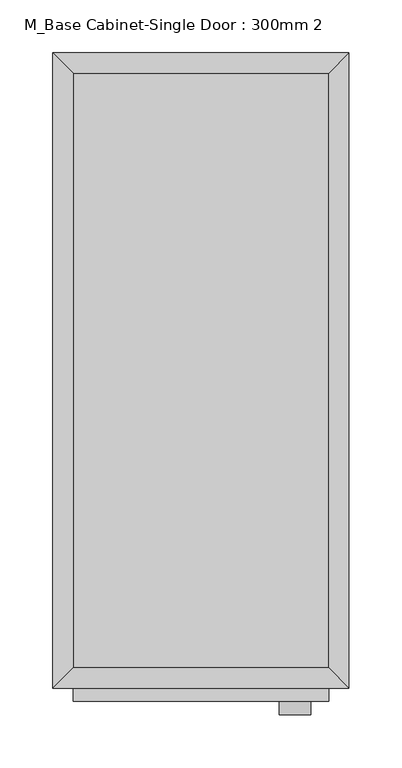
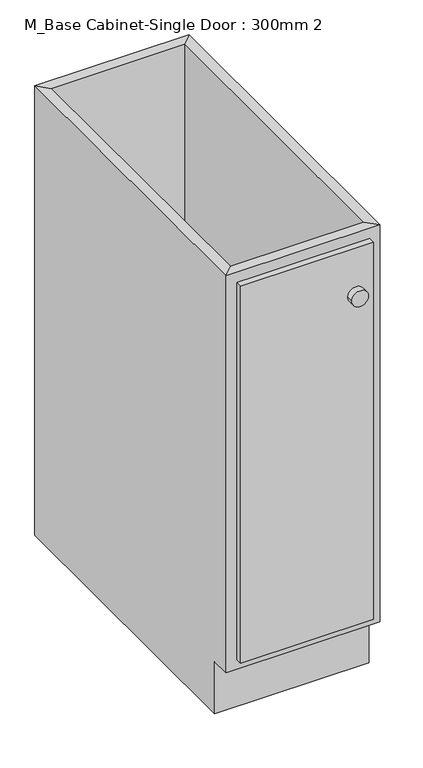
"""IFC4 building model written with IfcOpenShell, lengths in millimetres: furniture geometry, M_Base Cabinet-Single Door : 300mm 2."""

from ifc_helpers import new_model, si_unit, point, frame, frame_2d, origin, place, context, project, spatial, polyline, circle_curve, trimmed, segment, composite_curve, outline, extrude, faceted_brep, source, transform, mapped, element, save


def m_base_cabinet_single_door_300mm_2_1358b272(model_context):
    return source(origin(), model_context, "Body", "SolidModel", [
        faceted_brep([(139.3877049, -580.95, 860.0), (139.3877049, -580.95, 100.0), (-101.9122951, -580.95, 100.0), (-101.9122951, -580.95, 860.0), (-120.9622951, -600.0, 860.0), (158.4377049, -600.0, 860.0), (-120.9622951, -600.0, 100.0), (158.4377049, -600.0, 100.0), (-101.9122951, -565.0, 100.0), (-101.9122951, -19.05, 100.0), (-101.9122951, -19.05, 860.0), (-120.9622951, 0.0, 860.0), (-120.9622951, 0.0, 0.0), (-120.9622951, -565.0, 0.0), (-120.9622951, -565.0, 100.0), (139.3877049, -19.05, 100.0), (139.3877049, -19.05, 860.0), (158.4377049, 0.0, 860.0), (158.4377049, 0.0, 0.0), (139.3877049, -565.0, 100.0), (158.4377049, -565.0, 100.0), (158.4377049, -565.0, 0.0)], [[[0, 1, 2, 3]], [[0, 3, 4, 5]], [[5, 4, 6, 7]], [[2, 1, 7, 6]], [[3, 2, 8, 9, 10]], [[4, 3, 10, 11]], [[6, 4, 11, 12, 13, 14]], [[2, 6, 14, 8]], [[10, 9, 15, 16]], [[11, 10, 16, 17]], [[12, 11, 17, 18]], [[1, 0, 16, 15, 19]], [[0, 5, 17, 16]], [[5, 7, 20, 21, 18, 17]], [[7, 1, 19, 20]], [[8, 19, 15, 9]], [[18, 21, 13, 12]], [[13, 21, 20, 19, 8, 14]]]),
        extrude(outline(composite_curve([segment(trimmed(circle_curve(frame_2d((752.05, 107.6377049)), 15.0), [point((752.05, 92.6377049))], [point((752.05, 122.6377049))], False, "CARTESIAN"), True, "CONTINUOUS"), segment(trimmed(circle_curve(frame_2d((752.05, 107.6377049)), 15.0), [point((752.05, 122.6377049))], [point((752.05, 92.6377049))], False, "CARTESIAN"), True, "CONTINUOUS")], self_intersect=False)), frame((0.0, -625.4, 0.0), z_axis=(0.0, 1.0, 0.0), x_axis=(0.0, 0.0, 1.0)), (0.0, 0.0, 1.0), 12.7),
        extrude(outline(polyline([(139.3877049, -612.7), (-101.9122951, -612.7), (-101.9122951, -600.0), (139.3877049, -600.0), (139.3877049, -612.7)])), frame((0.0, 0.0, 119.05), z_axis=(0.0, 0.0, 1.0), x_axis=(1.0, 0.0, 0.0)), (0.0, 0.0, 1.0), 721.9),
        extrude(outline(polyline([(139.3877049, -19.05), (139.3877049, -580.95), (-101.9122951, -580.95), (-101.9122951, -19.05), (139.3877049, -19.05)])), frame((0.0, 0.0, 100.0), z_axis=(0.0, 0.0, 1.0), x_axis=(1.0, 0.0, 0.0)), (0.0, 0.0, 1.0), 19.05),
    ])


if __name__ == "__main__":
    model = new_model("IFC4")
    model_context = context("Model", 3, world=origin())
    ifc_project = project(units=[si_unit("LENGTHUNIT", "METRE", prefix="MILLI")], contexts=[model_context])
    site = spatial("IfcSite", under=ifc_project)
    building = spatial("IfcBuilding", under=site)
    placement = place(None, origin())
    m_base_cabinet_single_door_300mm_2_shape = m_base_cabinet_single_door_300mm_2_1358b272(model_context)
    element("IfcFurniture", 1, ObjectType="M_Base Cabinet-Single Door : 300mm 2", at=placement, inside=building, context=model_context, shape_type="MappedRepresentation", body=[
        mapped(m_base_cabinet_single_door_300mm_2_shape, transform((0.0, 0.0, 0.0), x_axis=(1.0, 0.0, 0.0), y_axis=(0.0, 1.0, 0.0), z_axis=(0.0, 0.0, 1.0))),
    ])
    save(model, "model.ifc")

# Revit data of these elements
# Type "M_Base Cabinet-Single Door : 300mm 2"
#   Depth = 1' - 11.62205"
#   Height = 2' - 9.85827"
#   Plinth Depth = 0' - 1.37795"
#   Plinth Height = 0' - 3.93701"
#   Width = 0' - 11"
#   Cabinet Material = Base cabinet 2120100 Aspekt - 83012120100 - White
#   Drawer Material = Base cabinet 2120100 Aspekt - 83012120100 - White
#   Handle Material = Cabinets - Handles
#   Default Elevation = 0
# Element 1 (IfcFurniture, "M_Base Cabinet-Single Door : 300mm 2")
#   Materials on its faces: "Base cabinet 2120100 Aspekt - 83012120100 - White", "Cabinets", "Cabinets - Handles"
# Materials
#   "Base cabinet 2120100 Aspekt - 83012120100 - White": class "Miscellaneous", colour RGB 255 255 255, transparency 0, Manufacturer = "Marbodal", URL = "http://www.marbodal.se", Cost = 0
#   "Cabinets - Handles": class "Metal", colour RGB 57 57 57, transparency 0
#   "Cabinets": class "Miscellaneous", colour RGB 249 249 249, transparency 0
